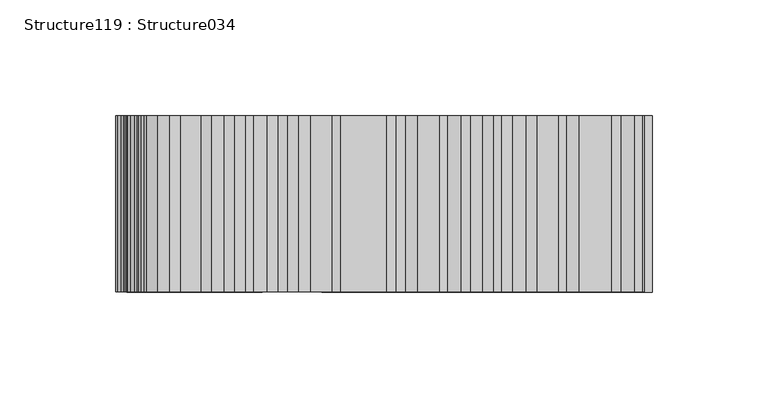
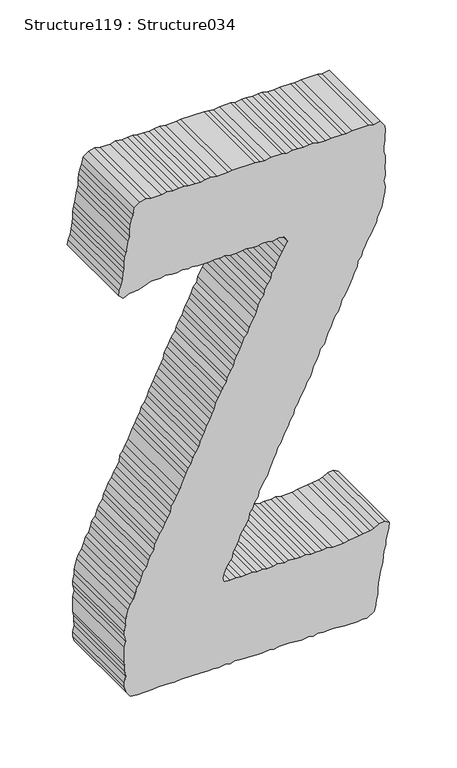
"""IFC4 building model written with IfcOpenShell, lengths in millimetres: proxy geometry, Structure119 : Structure034."""

from ifc_helpers import new_model, si_unit, frame, origin, place, context, project, spatial, polyline, outline, extrude, source, transform, mapped, element, save


def structure119_structure034_6e2f2597(model_context):
    return source(origin(), model_context, "Body", "SweptSolid", [
        extrude(outline(polyline([(3631.3410106, -45390.1637251), (3633.6821286, -45394.261885), (3633.0980525, -45398.9553531), (3630.7392839, -45403.0647453), (3629.5984101, -45406.5724107), (3628.998288, -45412.4324263), (3628.4158166, -45415.9577424), (3627.2396415, -45424.7317198), (3626.0554434, -45429.4251879), (3626.0554434, -45438.800892), (3627.2396415, -45443.4831279), (3626.0554434, -45447.584497), (3626.6571701, -45453.4525356), (3626.0554434, -45456.9682241), (3627.2396415, -45461.6536692), (3626.6571701, -45466.3359051), (3626.6571701, -45471.0293733), (3627.2396415, -45476.2956852), (3626.0554434, -45479.8113737), (3627.2396415, -45485.6713893), (3626.6571701, -45489.7807814), (3626.0554434, -45495.0470934), (3626.6571701, -45498.5724094), (3626.0554434, -45503.2482269), (3627.2396415, -45507.3560145), (3626.6571701, -45512.6335586), (3626.6571701, -45517.3061669), (3627.2396415, -45521.407536), (3626.6571701, -45526.6914986), (3627.2396415, -45531.9658336), (3630.7392839, -45533.1339857), (3634.2822506, -45531.9658336), (3639.5405396, -45530.1991641), (3642.4833842, -45528.4485405), (3647.1575971, -45524.9232245), (3651.2589662, -45524.3487761), (3655.3587307, -45521.9996351), (3660.0682449, -45519.6569125), (3665.3265338, -45517.898266), (3672.9435914, -45512.6335586), (3677.0449604, -45510.8652845), (3681.7271964, -45510.2812084), (3685.8285655, -45507.3560145), (3689.9540036, -45506.1718163), (3694.6298211, -45502.6641509), (3698.1294635, -45502.0800749), (3706.3289925, -45497.9803104), (3710.4560353, -45495.0470934), (3716.2887726, -45492.7043708), (3720.4158154, -45490.9553519), (3723.3313817, -45489.7807814), (3727.4311462, -45487.4300358), (3732.7167134, -45485.6713893), (3736.2163558, -45483.3382944), (3740.3161203, -45481.5700202), (3744.9999608, -45479.2272976), (3749.117376, -45476.8877843), (3753.2171405, -45475.7196322), (3758.485057, -45472.2039438), (3762.5848215, -45471.6102401), (3766.684586, -45468.6770231), (3771.3860772, -45466.9280042), (3775.4874463, -45464.5852816), (3779.5872107, -45462.234536), (3783.0868532, -45461.0695932), (3787.2042683, -45458.1363762), (3791.8865042, -45456.376125), (3795.4037973, -45455.2015545), (3800.6717138, -45452.2779651), (3804.7730829, -45450.5193186), (3809.4729695, -45449.3511665), (3812.3901405, -45445.8338735), (3821.1737455, -45442.9022611), (3825.849563, -45440.5595385), (3830.5574726, -45438.800892), (3834.6588416, -45437.0422455), (3838.1761347, -45434.1170515), (3843.432819, -45431.7679105), (3847.5598618, -45431.1838344), (3850.4754282, -45428.2490128), (3855.7353217, -45425.9175225), (3859.2606378, -45424.1492483), (3863.9332461, -45421.8081304), (3867.4601667, -45420.6303507), (3872.745734, -45417.7067613), (3877.4456205, -45417.1146622), (3880.9452629, -45414.1910728), (3885.6210804, -45413.0132931), (3889.7208449, -45410.6818028), (3893.822214, -45408.9151332), (3897.9476522, -45405.9883346), (3901.44569, -45404.2312927), (3906.7328618, -45401.2980757), (3911.4054701, -45400.7220227), (3919.6066036, -45396.6126306), (3928.4158823, -45394.8555887), (3931.9058971, -45394.261885), (3937.1930689, -45393.6810182), (3942.4770315, -45394.8555887), (3947.1496398, -45393.6810182), (3950.0940891, -45393.6810182), (3954.7506513, -45394.261885), (3960.0602876, -45393.6810182), (3964.7361051, -45393.6810182), (3968.8198235, -45394.8555887), (3974.1214368, -45394.8555887), (3978.8036727, -45394.261885), (3982.8793681, -45394.261885), (3988.1633307, -45393.6810182), (3992.2614906, -45394.261885), (3997.5486624, -45397.7807827), (3996.390138, -45403.6472167), (3997.5486624, -45407.7469812), (3997.5486624, -45421.8081304), (3996.390138, -45427.092093), (3996.9645864, -45430.5997584), (3996.9645864, -45439.9658348), (3996.390138, -45444.659303), (3996.390138, -45450.5193186), (3997.5486624, -45455.2015545), (3997.5486624, -45458.7188476), (3996.9645864, -45463.4123157), (3997.5486624, -45468.6770231), (3997.5486624, -45472.7783922), (3996.390138, -45478.6464308), (3997.5486624, -45482.1637239), (3997.5486624, -45491.5298003), (3996.390138, -45496.8057399), (3996.9645864, -45500.915132), (3997.5486624, -45505.0148965), (3997.5486624, -45524.9232245), (3996.9645864, -45528.4485405), (3996.9645864, -45537.8162216), (3997.5486624, -45543.1017888), (3996.9645864, -45547.7760017), (3996.390138, -45551.8757662), (3996.390138, -45556.5692343), (3996.9645864, -45562.4260407), (3997.5486624, -45565.9529614), (3997.5486624, -45570.6287789), (3996.9645864, -45575.3222471), (3997.5486624, -45580.5965821), (3996.390138, -45585.278818), (3996.390138, -45594.0736552), (3997.5486624, -45598.7558911), (3996.390138, -45604.0222031), (3992.8375436, -45608.7156712), (3987.0048063, -45609.8902417), (3983.4794902, -45611.0664168), (3978.8036727, -45612.2313597), (3974.1214368, -45612.8250633), (3968.8198235, -45612.8250633), (3964.7361051, -45613.9900062), (3954.7506513, -45615.7486527), (3951.2606365, -45616.9248278), (3946.5511223, -45617.5072993), (3940.718385, -45617.5072993), (3937.1930689, -45618.0993983), (3931.3346579, -45618.6754513), (3926.6492128, -45619.8500218), (3922.5494483, -45621.6070638), (3917.8479571, -45622.2007674), (3914.3499193, -45618.0993983), (3916.6653636, -45613.4059302), (3917.2735087, -45609.3077703), (3917.8479571, -45604.6143021), (3919.0321552, -45600.5145377), (3921.3748778, -45594.654522), (3921.3748778, -45586.4549931), (3922.5494483, -45582.3552286), (3921.3748778, -45576.4968176), (3921.3748778, -45572.3954485), (3922.5494483, -45567.7035849), (3921.3748778, -45562.4260407), (3922.5494483, -45559.4944283), (3921.3748778, -45554.2361394), (3921.3748778, -45544.2587086), (3921.9733953, -45540.7510432), (3921.9733953, -45534.8926322), (3922.5494483, -45530.7912631), (3921.3748778, -45526.6914986), (3921.3748778, -45521.407536), (3921.9733953, -45516.7333231), (3922.5494483, -45513.2144255), (3921.3748778, -45507.9400905), (3921.3748778, -45503.8387214), (3922.5494483, -45499.1468579), (3922.5494483, -45495.0470934), (3921.3748778, -45490.3616482), (3922.5494483, -45485.0873133), (3921.3748778, -45480.3954497), (3916.6653636, -45477.4702557), (3912.5896682, -45479.8113737), (3909.0627475, -45482.1637239), (3904.9645876, -45483.9127428), (3900.2887701, -45486.8459598), (3895.5888836, -45488.6046063), (3892.6636896, -45490.9553519), (3887.9621984, -45491.5298003), (3883.8881076, -45494.4630173), (3879.7610648, -45496.8057399), (3875.0772243, -45497.397839), (3871.5599312, -45500.3214283), (3867.4601667, -45502.6641509), (3862.2018778, -45503.8387214), (3857.5019912, -45506.1718163), (3850.4754282, -45510.2812084), (3845.1914656, -45511.4557789), (3842.2758992, -45514.3825775), (3837.6000817, -45516.1492471), (3833.4730389, -45517.898266), (3828.2163546, -45520.831483), (3824.1149855, -45522.5837111), (3820.015221, -45523.7663046), (3816.4883003, -45526.1010042), (3811.2043377, -45529.0245936), (3807.714323, -45529.6166926), (3803.0064134, -45533.1339857), (3800.0876378, -45534.3085562), (3795.4037973, -45536.6416511), (3791.3056374, -45539.0020243), (3786.6298199, -45540.1589442), (3783.0868532, -45541.9256137), (3778.4046172, -45543.6746326), (3773.7015215, -45546.6190819), (3769.0176809, -45548.3681008), (3765.5019925, -45550.1267473), (3761.418274, -45552.4694698), (3757.3185096, -45553.6440403), (3752.6170184, -45555.9867629), (3749.117376, -45558.9103523), (3743.8414364, -45560.0865274), (3740.9162424, -45562.4260407), (3736.7988273, -45564.1846873), (3732.7167134, -45565.9529614), (3723.9154578, -45570.0447029), (3719.2316172, -45572.3954485), (3714.5301261, -45574.738171), (3711.6145597, -45577.0889166), (3706.3289925, -45577.6617604), (3702.229228, -45580.012506), (3698.1294635, -45582.3552286), (3694.029699, -45584.1138751), (3689.9540036, -45587.0374645), (3684.6443673, -45589.3801871), (3681.7271964, -45591.1388336), (3677.0449604, -45591.7309326), (3672.3691429, -45595.2482257), (3669.4262983, -45596.4067501), (3663.5598643, -45598.1718151), (3660.6250426, -45601.0970091), (3656.5429288, -45602.2715796), (3651.2589662, -45604.0222031), (3648.3161216, -45606.3729487), (3643.0578326, -45608.1315952), (3638.3563415, -45609.8902417), (3634.2822506, -45612.2313597), (3630.7392839, -45613.9900062), (3622.555801, -45616.3327288), (3617.8559144, -45616.3327288), (3612.0135494, -45617.5072993), (3608.4705827, -45617.5072993), (3602.6298224, -45616.3327288), (3597.9540049, -45617.5072993), (3583.8864372, -45617.5072993), (3580.3691442, -45616.9248278), (3575.6853037, -45616.9248278), (3570.9854171, -45616.3327288), (3565.7094775, -45617.5072993), (3561.6257591, -45617.5072993), (3556.9258725, -45616.3327288), (3551.6675836, -45612.2313597), (3551.0658569, -45606.3729487), (3551.0658569, -45592.8958755), (3551.6675836, -45588.2136396), (3551.6675836, -45578.2458365), (3551.0658569, -45574.738171), (3551.6675836, -45568.8781554), (3551.6675836, -45551.2932948), (3551.0658569, -45546.6190819), (3551.6675836, -45541.3351193), (3551.0658569, -45536.6416511), (3552.242032, -45530.7912631), (3551.0658569, -45526.6914986), (3552.242032, -45522.5837111), (3551.6675836, -45517.3061669), (3551.6675836, -45508.5321895), (3551.0658569, -45503.8387214), (3551.0658569, -45498.5724094), (3552.242032, -45493.2980745), (3551.0658569, -45489.1870777), (3552.242032, -45484.5048418), (3552.242032, -45475.7196322), (3551.0658569, -45465.7534337), (3552.242032, -45459.8950227), (3551.0658569, -45455.2015545), (3552.242032, -45451.6938891), (3551.6675836, -45447.000421), (3552.242032, -45441.734109), (3552.242032, -45437.6327399), (3551.0658569, -45428.2490128), (3551.0658569, -45417.7067613), (3551.6675836, -45413.6069968), (3551.0658569, -45409.4976047), (3555.1848766, -45403.0647453), (3561.025637, -45401.8789425), (3565.1254015, -45401.2980757), (3569.8268927, -45400.1299236), (3573.9266571, -45400.1299236), (3579.7690221, -45399.5458476), (3584.4689087, -45398.9553531), (3589.1527492, -45397.7807827), (3592.6700423, -45397.2063342), (3597.3538828, -45396.0285545), (3602.6298224, -45395.4476877), (3606.7295868, -45394.8555887), (3612.0135494, -45393.1049652), (3616.69739, -45393.1049652), (3621.3732075, -45391.9303947), (3626.0554434, -45390.7542196), (3631.3410106, -45390.1637251)])), frame((0.0, 247945.1599557, 0.0), z_axis=(0.0, 1.0, 0.0), x_axis=(0.0, 0.0, 1.0)), (0.0, 0.0, 1.0), 76.2),
    ])


if __name__ == "__main__":
    model = new_model("IFC4")
    model_context = context("Model", 3, world=origin())
    ifc_project = project(units=[si_unit("LENGTHUNIT", "METRE", prefix="MILLI")], contexts=[model_context])
    site = spatial("IfcSite", under=ifc_project)
    building = spatial("IfcBuilding", under=site)
    placement = place(None, origin())
    structure119_structure034_shape = structure119_structure034_6e2f2597(model_context)
    element("IfcBuildingElementProxy", 1, Name="Structure119 : Structure034", ObjectType="Structure119 : Structure034", at=placement, inside=building, context=model_context, shape_type="MappedRepresentation", body=[
        mapped(structure119_structure034_shape, transform((0.0, 0.0, 0.0), x_axis=(1.0, 0.0, 0.0), y_axis=(0.0, 1.0, 0.0), z_axis=(0.0, 0.0, 1.0))),
    ])
    save(model, "model.ifc")

# Revit data of these elements
# Type "Structure119 : Structure034"
#   NameOverride = "Structure034"
# Element 1 (IfcBuildingElementProxy, "Structure119 : Structure034")
#   Materials on its faces: "BRUSHED ALUM. LETTERING"
# Materials
#   "BRUSHED ALUM. LETTERING": class "Unassigned", colour RGB 169 181 186, transparency 0, Cost = 0
